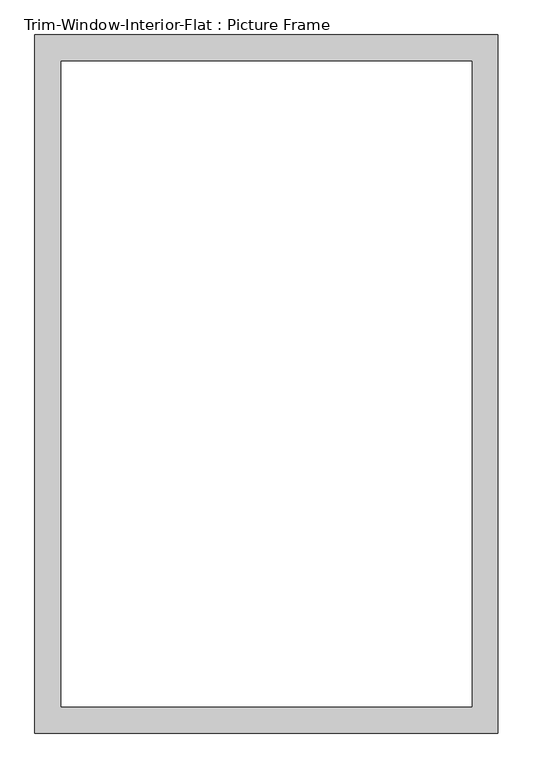
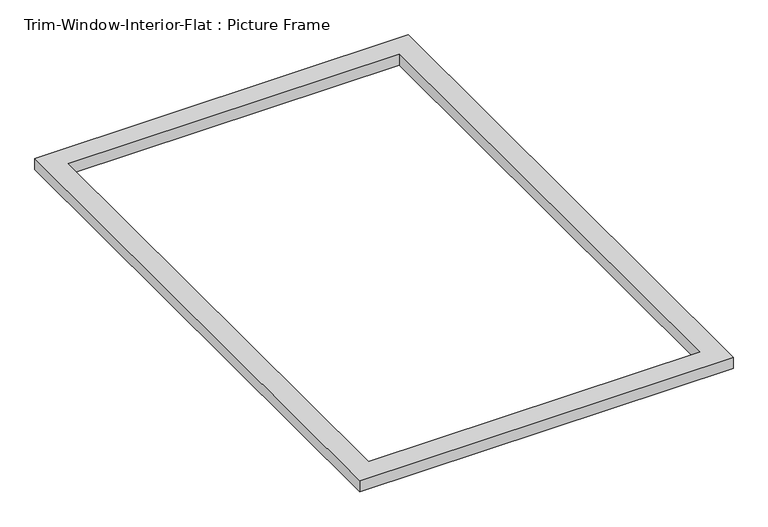
"""IFC4 building model written with IfcOpenShell, lengths in millimetres: proxy geometry, Trim-Window-Interior-Flat : Picture Frame."""

import ifcopenshell
import ifcopenshell.guid

model = None  # the IFC model being written
_history = None  # IfcOwnerHistory: only IFC2X3 demands one
_inside = {}  # id of a spatial element -> (the spatial element, [elements in it])
_under = {}  # id of a project, library or spatial element -> (it, [spatial elements below it])
_declared = {}  # id of a project -> (the project, [libraries it declares])
_typed = {}  # id of a type object -> (the type object, [elements of that type])
_made_of = {}  # id of a material, layer set ... -> (it, [elements and type objects made of it])


def new_model(schema):
    """Start an empty IFC model of exactly this schema.

    Asked for "IFC4X3", IfcOpenShell would pick the latest addendum, in which some entities
    have other attributes; the version numbers below select the first issue.
    IFC2X3 requires an IfcOwnerHistory on every rooted entity: one is made here for all.
    """
    global model, _history
    if schema == "IFC4X3":
        model = ifcopenshell.file(schema_version=(4, 3, 0, 0))
    else:
        model = ifcopenshell.file(schema=schema)
    _inside.clear()
    _under.clear()
    _declared.clear()
    _typed.clear()
    _made_of.clear()
    _history = None
    if model.schema == "IFC2X3":
        org = make("IfcOrganization", Name="unknown")
        user = make(
            "IfcPersonAndOrganization",
            ThePerson=make("IfcPerson", FamilyName="unknown"),
            TheOrganization=org,
        )
        app = make(
            "IfcApplication",
            ApplicationDeveloper=org,
            Version="unknown",
            ApplicationFullName="unknown",
            ApplicationIdentifier="unknown",
        )
        _history = make(
            "IfcOwnerHistory",
            OwningUser=user,
            OwningApplication=app,
            ChangeAction="ADDED",
            CreationDate=0,
        )
    return model


def make(cls, **values):
    """One entity of the class cls with the attributes given. An attribute that is None is left unset."""
    return model.create_entity(
        cls, **{name: value for name, value in values.items() if value is not None}
    )


def rooted(cls, **values):
    """An entity with a GlobalId (a new one), such as an element, a storey or a relation."""
    return make(cls, GlobalId=ifcopenshell.guid.new(), OwnerHistory=_history, **values)


def si_unit(unit_type, name, prefix=None):
    """IfcSIUnit, for example si_unit("LENGTHUNIT", "METRE", prefix="MILLI")."""
    return make("IfcSIUnit", UnitType=unit_type, Prefix=prefix, Name=name)


def assignment(units):
    """IfcUnitAssignment: the units of a project."""
    return None if units is None else make("IfcUnitAssignment", Units=units)


def point(xyz):
    """IfcCartesianPoint."""
    return None if xyz is None else make("IfcCartesianPoint", Coordinates=xyz)


def direction(xyz):
    """IfcDirection."""
    return None if xyz is None else make("IfcDirection", DirectionRatios=xyz)


def frame(location, z_axis=None, x_axis=None):
    """IfcAxis2Placement3D, a coordinate frame: its origin and axes. An axis left out is left unset."""
    return make(
        "IfcAxis2Placement3D",
        Location=point(location),
        Axis=direction(z_axis),
        RefDirection=direction(x_axis),
    )


def origin():
    """The frame at (0, 0, 0) with its axes left unset."""
    return frame((0.0, 0.0, 0.0))


def origin_with_axes():
    """The frame at (0, 0, 0) with the z axis (0, 0, 1) and the x axis (1, 0, 0) written out."""
    return frame((0.0, 0.0, 0.0), z_axis=(0.0, 0.0, 1.0), x_axis=(1.0, 0.0, 0.0))


def place(relative_to, where):
    """IfcLocalPlacement: puts the frame where relative to a parent placement (None: the world)."""
    return make(
        "IfcLocalPlacement", PlacementRelTo=relative_to, RelativePlacement=where
    )


def context(
    kind, dimensions, precision=None, world=None, true_north=None, identifier=None
):
    """IfcGeometricRepresentationContext, for example the 3D "Model" context."""
    return make(
        "IfcGeometricRepresentationContext",
        ContextIdentifier=identifier,
        ContextType=kind,
        CoordinateSpaceDimension=dimensions,
        Precision=precision,
        WorldCoordinateSystem=world,
        TrueNorth=true_north,
    )


def project(units=None, contexts=None):
    """IfcProject with its units and contexts."""
    return rooted(
        "IfcProject",
        Name="project",
        RepresentationContexts=contexts,
        UnitsInContext=assignment(units),
    )


def spatial(cls, under=None, at=None, **own):
    """A site, building, storey or space (cls), placed at a placement, below another one or the project."""
    s = rooted(cls, ObjectPlacement=at, **own)
    if under is not None:
        _under.setdefault(under.id(), (under, []))[1].append(s)
    return s


def polyline(points):
    """IfcPolyline through the points."""
    return make("IfcPolyline", Points=[point(p) for p in points])


def outline(outer, holes=None, kind="AREA"):
    """IfcArbitraryClosedProfileDef: a profile drawn as a closed curve; with holes, ...WithVoids."""
    if holes is None:
        return make("IfcArbitraryClosedProfileDef", ProfileType=kind, OuterCurve=outer)
    return make(
        "IfcArbitraryProfileDefWithVoids",
        ProfileType=kind,
        OuterCurve=outer,
        InnerCurves=holes,
    )


def extrude(swept, where, along, depth):
    """IfcExtrudedAreaSolid: the profile swept, set in the frame where, extruded along a direction by depth."""
    return make(
        "IfcExtrudedAreaSolid",
        SweptArea=swept,
        Position=where,
        ExtrudedDirection=direction(along),
        Depth=depth,
    )


def shape(context_of_items, identifier, shape_type, items):
    """IfcShapeRepresentation: the items that make up one representation, for example the "Body"."""
    return make(
        "IfcShapeRepresentation",
        ContextOfItems=context_of_items,
        RepresentationIdentifier=identifier,
        RepresentationType=shape_type,
        Items=items,
    )


def source(mapping_origin, context_of_items, identifier, shape_type, items):
    """IfcRepresentationMap: a shape defined once, which mapped items show again and again."""
    return make(
        "IfcRepresentationMap",
        MappingOrigin=mapping_origin,
        MappedRepresentation=shape(context_of_items, identifier, shape_type, items),
    )


def transform(
    local_origin,
    x_axis=None,
    y_axis=None,
    z_axis=None,
    scale=None,
    scale2=None,
    scale3=None,
    uniform=True,
):
    """IfcCartesianTransformationOperator3D, or its non-uniform kind. x_axis, y_axis, z_axis: its Axis1, 2, 3."""
    if uniform:
        return make(
            "IfcCartesianTransformationOperator3D",
            Axis1=direction(x_axis),
            Axis2=direction(y_axis),
            LocalOrigin=point(local_origin),
            Scale=scale,
            Axis3=direction(z_axis),
        )
    return make(
        "IfcCartesianTransformationOperator3DnonUniform",
        Axis1=direction(x_axis),
        Axis2=direction(y_axis),
        LocalOrigin=point(local_origin),
        Scale=scale,
        Axis3=direction(z_axis),
        Scale2=scale2,
        Scale3=scale3,
    )


def mapped(mapping_source, mapping_target):
    """IfcMappedItem: shows the shape of a source again, moved by a transform."""
    return make(
        "IfcMappedItem", MappingSource=mapping_source, MappingTarget=mapping_target
    )


def made_of(thing, what):
    """Note that an element or type object is made of a material, layer set ...; save() writes the relation."""
    if what is not None:
        _made_of.setdefault(what.id(), (what, []))[1].append(thing)
    return thing


def element(
    cls,
    number,
    at=None,
    inside=None,
    cuts=None,
    type_object=None,
    material=None,
    context=None,
    identifier="Body",
    shape_type=None,
    held_by="IfcProductDefinitionShape",
    body=None,
    shapes=None,
    **own,
):
    """One element of the class cls, such as IfcWall. Its Tag is "e" and its number.

    at: its placement. inside: the storey or other place that contains it. cuts: it is an
    opening in that element (IfcRelVoidsElement). A single representation is given by context,
    identifier, shape_type and body (its items); several are given by shapes. held_by: the class
    of the entity that holds the representations. save() writes the other relations.
    """
    e = rooted(cls, Tag="e%d" % number, ObjectPlacement=at, **own)
    if body is not None:
        shapes = [shape(context, identifier, shape_type, body)]
    if shapes is not None:
        e.Representation = make(held_by, Representations=shapes)
    if inside is not None:
        _inside.setdefault(inside.id(), (inside, []))[1].append(e)
    if cuts is not None:
        rooted(
            "IfcRelVoidsElement", RelatingBuildingElement=cuts, RelatedOpeningElement=e
        )
    if type_object is not None:
        _typed.setdefault(type_object.id(), (type_object, []))[1].append(e)
    return made_of(e, material)


def aggregate(whole, parts):
    """IfcRelAggregates: a whole, such as a stair, and the parts it consists of."""
    return rooted("IfcRelAggregates", RelatingObject=whole, RelatedObjects=parts)


def save(model, path):
    """Write the relations noted so far, then the file.

    IfcRelAggregates (storeys below a building ...), IfcRelContainedInSpatialStructure (elements
    in a storey), IfcRelDefinesByType, IfcRelAssociatesMaterial and IfcRelDeclares: one each for
    every whole, place, type object, material and project.
    """
    for whole, parts in _under.values():
        aggregate(whole, parts)
    for where, things in _inside.values():
        rooted(
            "IfcRelContainedInSpatialStructure",
            RelatedElements=things,
            RelatingStructure=where,
        )
    for kind, things in _typed.values():
        rooted("IfcRelDefinesByType", RelatedObjects=things, RelatingType=kind)
    for what, things in _made_of.values():
        rooted("IfcRelAssociatesMaterial", RelatedObjects=things, RelatingMaterial=what)
    for by, libraries in _declared.values():
        rooted("IfcRelDeclares", RelatingContext=by, RelatedDefinitions=libraries)
    model.write(path)


def trim_window_interior_flat_picture_frame_99361138(model_context):
    return source(origin(), model_context, "Body", "SweptSolid", [
        extrude(outline(polyline([(501.65, 44.45), (501.65, -1466.85), (-501.65, -1466.85), (-501.65, 44.45), (501.65, 44.45)]), holes=[polyline([(444.5, -12.7), (-444.5, -12.7), (-444.5, -1409.7), (444.5, -1409.7), (444.5, -12.7)])]), origin_with_axes(), (0.0, 0.0, 1.0), 31.75),
    ])


if __name__ == "__main__":
    model = new_model("IFC4")
    model_context = context("Model", 3, world=origin())
    ifc_project = project(units=[si_unit("LENGTHUNIT", "METRE", prefix="MILLI")], contexts=[model_context])
    site = spatial("IfcSite", under=ifc_project)
    building = spatial("IfcBuilding", under=site)
    placement = place(None, origin())
    trim_window_interior_flat_picture_frame_shape = trim_window_interior_flat_picture_frame_99361138(model_context)
    element("IfcBuildingElementProxy", 1, Name="Trim-Window-Interior-Flat : Picture Frame", ObjectType="Trim-Window-Interior-Flat : Picture Frame", at=placement, inside=building, context=model_context, shape_type="MappedRepresentation", body=[
        mapped(trim_window_interior_flat_picture_frame_shape, transform((0.0, 0.0, 0.0), x_axis=(1.0, 0.0, 0.0), y_axis=(0.0, 1.0, 0.0), z_axis=(0.0, 0.0, 1.0))),
    ])
    save(model, "model.ifc")

# Revit data of these elements
# Type "Trim-Window-Interior-Flat : Picture Frame"
#   Trim Thickness_Picture Frame = 0' - 1 1/4"
#   Trim Width = 0' - 2 1/4"
#   Trim Thickness_with Sill = 0' - 0 3/4"
#   Sill Thickness = 0' - 1 1/4"
#   Opening Width [instance default] = 2' - 0"
#   Opening Height [instance default] = 3' - 0"
#   Default Elevation = 4' - 0"
#   Sill = no
#   Picture Frame = yes
#   Trim Material [instance default] = none
# Element 1 (IfcBuildingElementProxy, "Trim-Window-Interior-Flat : Picture Frame")
#   Opening Width = 3' - 0"
#   Opening Height = 4' - 8"
#   Trim Material = Wood - Stained
#   Materials on its faces: "Wood - Stained"
# Materials
#   "Wood - Stained": class "Wood", colour RGB 224 178 126, transparency 0, Cost = 0
